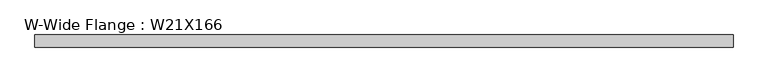
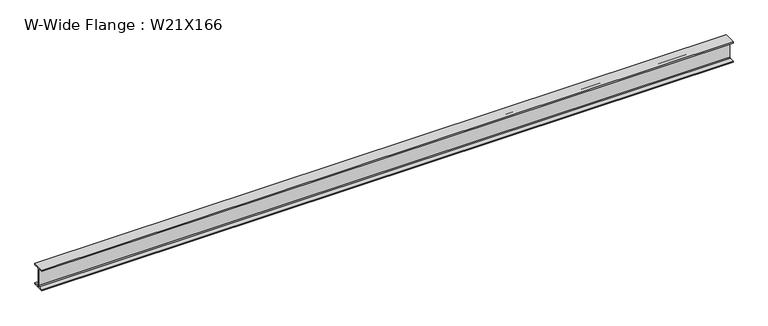
"""IFC4 building model written with IfcOpenShell, lengths in millimetres: beam geometry, W-Wide Flange : W21X166."""

from ifc_helpers import new_model, si_unit, point, frame, frame_2d, origin, place, context, project, spatial, polyline, circle_curve, trimmed, segment, composite_curve, outline, extrude, source, transform, mapped, element, save


def w_wide_flange_w21x166_4fa183b2(model_context):
    return source(origin(), model_context, "Body", "SweptSolid", [
        extrude(outline(composite_curve([segment(polyline([(157.48, -251.206), (157.48, -285.75), (-157.48, -285.75), (-157.48, -251.206), (-32.131, -251.206)]), True, "CONTINUOUS"), segment(trimmed(circle_curve(frame_2d((-32.131, -228.6)), 22.606), [point((-32.131, -251.206))], [point((-9.525, -228.6))], True, "CARTESIAN"), True, "CONTINUOUS"), segment(polyline([(-9.525, -228.6), (-9.525, 228.6)]), True, "CONTINUOUS"), segment(trimmed(circle_curve(frame_2d((-32.131, 228.6)), 22.606), [point((-9.525, 228.6))], [point((-32.131, 251.206))], True, "CARTESIAN"), True, "CONTINUOUS"), segment(polyline([(-32.131, 251.206), (-157.48, 251.206), (-157.48, 285.75), (157.48, 285.75), (157.48, 251.206), (32.131, 251.206)]), True, "CONTINUOUS"), segment(trimmed(circle_curve(frame_2d((32.131, 228.6)), 22.606), [point((32.131, 251.206))], [point((9.525, 228.6))], True, "CARTESIAN"), True, "CONTINUOUS"), segment(polyline([(9.525, 228.6), (9.525, -228.6)]), True, "CONTINUOUS"), segment(trimmed(circle_curve(frame_2d((32.131, -228.6)), 22.606), [point((9.525, -228.6))], [point((32.131, -251.206))], True, "CARTESIAN"), True, "CONTINUOUS"), segment(polyline([(32.131, -251.206), (157.48, -251.206)]), True, "CONTINUOUS")], self_intersect=False)), frame((-9137.6596451, 0.0, 0.0), z_axis=(1.0, 0.0, 0.0), x_axis=(0.0, 1.0, 0.0)), (0.0, 0.0, 1.0), 18150.0379668),
    ])


if __name__ == "__main__":
    model = new_model("IFC4")
    model_context = context("Model", 3, world=origin())
    ifc_project = project(units=[si_unit("LENGTHUNIT", "METRE", prefix="MILLI")], contexts=[model_context])
    site = spatial("IfcSite", under=ifc_project)
    building = spatial("IfcBuilding", under=site)
    placement = place(None, origin())
    w_wide_flange_w21x166_shape = w_wide_flange_w21x166_4fa183b2(model_context)
    element("IfcBeam", 1, ObjectType="W-Wide Flange : W21X166", at=placement, inside=building, context=model_context, shape_type="MappedRepresentation", body=[
        mapped(w_wide_flange_w21x166_shape, transform((0.0, 0.0, 0.0), x_axis=(1.0, 0.0, 0.0), y_axis=(0.0, 1.0, 0.0), z_axis=(0.0, 0.0, 1.0))),
    ])
    save(model, "model.ifc")

# Revit data of these elements
# Type "W-Wide Flange : W21X166"
#   Assembly Code = "B10"
#   W = 166
#   Length [instance default] = 5' - 0"
#   bf = 1' - 0.4"
#   d = 1' - 10 1/2"
#   k = 0' - 2 1/4"
#   k2 = 0' - 0.89"
#   tf = 0' - 1.36"
#   tw = 0' - 0 3/4"
#   A = 0.338889 SF
#   Structural Material [instance default] = Steel ASTM A992
# Element 1 (IfcBeam, "W-Wide Flange : W21X166")
#   Structural Material = Steel
#   Materials on its faces: "Steel"
# Materials
#   "Steel ASTM A992": class "Metal", colour RGB 199 199 199, transparency 0, Description = "Structural steel 50ksi", Cost = 0
#   "Steel": class "Metal", colour RGB 118 118 114, transparency 0, Description = "Steel, mill finish", Cost = 0
